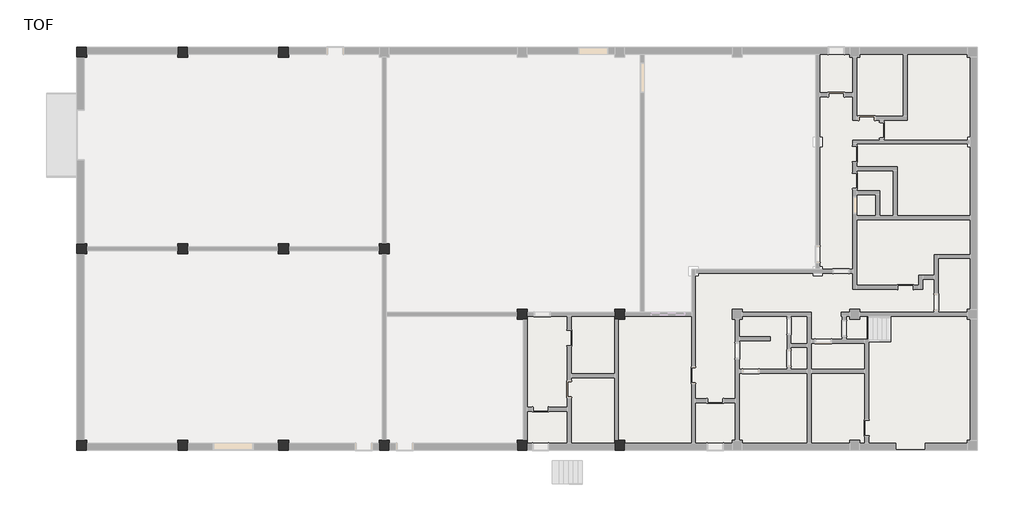
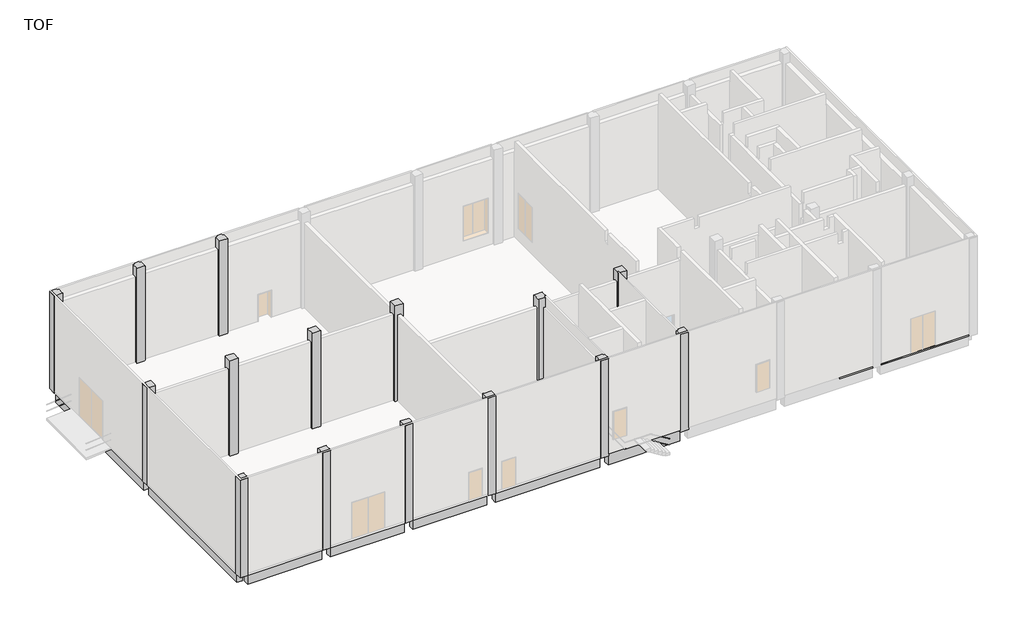
# One storey, part 4 of 5: 15 columns, 9 beams, 4 slabs.
"""IFC4 building model written with IfcOpenShell, lengths in millimetres."""

from ifc_helpers import new_model, si_unit, frame, origin, place, context, project, spatial, polyline, outline, extrude, faceted_brep, element, save

model = new_model("IFC4")

# Units and contexts
model_context = context("Model", 3, world=origin())
ifc_project = project(units=[si_unit("LENGTHUNIT", "METRE", prefix="MILLI")], contexts=[model_context])

# Site, building, storey
site = spatial("IfcSite", under=ifc_project)
building = spatial("IfcBuilding", under=site)
storey = spatial("IfcBuildingStorey", under=building, Name="TOF", Elevation=150.0)

# Beams
placement = place(None, origin())
element("IfcBeam", 1, ObjectType="RC Beam_Rectangular : H_SB_ACB_B400xH900", at=placement, inside=storey, context=model_context, shape_type="SweptSolid", body=[
    extrude(outline(polyline([(124.7, 12616.5208589), (-275.3, 12616.5208589), (-275.3, 23716.5208589), (124.7, 23716.5208589), (124.7, 12616.5208589)])), frame((0.0, 0.0, -750.0), z_axis=(0.0, 0.0, 1.0), x_axis=(1.0, 0.0, 0.0)), (0.0, 0.0, 1.0), 800.0),
])
element("IfcBeam", 2, ObjectType="RC Beam_Rectangular : H_SB_ACB_B400xH900", at=placement, inside=storey, context=model_context, shape_type="SweptSolid", body=[
    extrude(outline(polyline([(124.7, 916.5208589), (-275.3, 916.5208589), (-275.3, 12016.5208589), (124.7, 12016.5208589), (124.7, 916.5208589)])), frame((0.0, 0.0, -750.0), z_axis=(0.0, 0.0, 1.0), x_axis=(1.0, 0.0, 0.0)), (0.0, 0.0, 1.0), 750.0),
])
element("IfcBeam", 3, ObjectType="RC Beam_Rectangular : H_SB_ACB_B400xH900", at=placement, inside=storey, context=model_context, shape_type="SweptSolid", body=[
    extrude(outline(polyline([(5624.7, 24216.5208589), (5624.7, 23816.5208589), (224.7, 23816.5208589), (224.7, 24216.5208589), (5624.7, 24216.5208589)])), frame((0.0, 0.0, -750.0), z_axis=(0.0, 0.0, 1.0), x_axis=(1.0, 0.0, 0.0)), (0.0, 0.0, 1.0), 800.0),
])
element("IfcBeam", 4, ObjectType="RC Beam_Rectangular : H_SB_ACB_B400xH900", at=placement, inside=storey, context=model_context, shape_type="SweptSolid", body=[
    extrude(outline(polyline([(11624.7, 24216.5208589), (11624.7, 23816.5208589), (6224.7, 23816.5208589), (6224.7, 24216.5208589), (11624.7, 24216.5208589)])), frame((0.0, 0.0, -750.0), z_axis=(0.0, 0.0, 1.0), x_axis=(1.0, 0.0, 0.0)), (0.0, 0.0, 1.0), 800.0),
])
element("IfcBeam", 5, ObjectType="RC Beam_Rectangular : H_SB_ACB_B400xH900", at=placement, inside=storey, context=model_context, shape_type="SweptSolid", body=[
    extrude(outline(polyline([(5624.7, 816.5208589), (5624.7, 416.5208589), (224.7, 416.5208589), (224.7, 816.5208589), (5624.7, 816.5208589)])), frame((0.0, 0.0, -750.0), z_axis=(0.0, 0.0, 1.0), x_axis=(1.0, 0.0, 0.0)), (0.0, 0.0, 1.0), 750.0),
])
element("IfcBeam", 6, ObjectType="RC Beam_Rectangular : H_SB_ACB_B400xH900", at=placement, inside=storey, context=model_context, shape_type="SweptSolid", body=[
    extrude(outline(polyline([(11624.7, 816.5208589), (11624.7, 416.5208589), (6224.7, 416.5208589), (6224.7, 816.5208589), (11624.7, 816.5208589)])), frame((0.0, 0.0, -750.0), z_axis=(0.0, 0.0, 1.0), x_axis=(1.0, 0.0, 0.0)), (0.0, 0.0, 1.0), 750.0),
])
element("IfcBeam", 7, ObjectType="RC Beam_Rectangular : H_SB_ACB_B400xH900", at=placement, inside=storey, context=model_context, shape_type="SweptSolid", body=[
    extrude(outline(polyline([(17624.7, 816.5208589), (17624.7, 416.5208589), (12224.7, 416.5208589), (12224.7, 816.5208589), (17624.7, 816.5208589)])), frame((0.0, 0.0, -750.0), z_axis=(0.0, 0.0, 1.0), x_axis=(1.0, 0.0, 0.0)), (0.0, 0.0, 1.0), 750.0),
])
element("IfcBeam", 8, ObjectType="RC Beam_Rectangular : H_SB_ACB_B400xH900", at=placement, inside=storey, context=model_context, shape_type="SweptSolid", body=[
    extrude(outline(polyline([(25824.7, 816.5208589), (25824.7, 416.5208589), (18224.7, 416.5208589), (18224.7, 816.5208589), (25824.7, 816.5208589)])), frame((0.0, 0.0, -750.0), z_axis=(0.0, 0.0, 1.0), x_axis=(1.0, 0.0, 0.0)), (0.0, 0.0, 1.0), 750.0),
])
element("IfcBeam", 9, ObjectType="RC Beam_Rectangular : H_SB_ACB_B400xH900", at=placement, inside=storey, context=model_context, shape_type="Brep", body=[
    faceted_brep([(26424.7, 816.5208589, 150.0), (26424.7, 746.5208589, 150.0), (26424.7, 416.5208589, 150.0), (31624.7, 416.5208589, 150.0), (31624.7, 746.5208589, 150.0), (31624.7, 816.5208589, 150.0), (26424.7, 416.5208589, -750.0), (31624.7, 416.5208589, -750.0), (26424.7, 816.5208589, -750.0), (31624.7, 816.5208589, -750.0)], [[[0, 1, 2, 3, 4, 5]], [[2, 6, 7, 3]], [[6, 8, 9, 7]], [[8, 0, 5, 9]], [[2, 1, 0, 8, 6]], [[5, 4, 3, 7, 9]]]),
])

# Columns
element("IfcColumn", 10, ObjectType="RC_Column_Rectangular : H_SC_ACC_W600xL600", at=placement, inside=storey, context=model_context, shape_type="Brep", body=[
    faceted_brep([(224.7, 12616.5208589, 0.0), (224.7, 12316.5208589, 0.0), (224.7, 12016.5208589, 0.0), (-375.3, 12016.5208589, 0.0), (-375.3, 12616.5208589, 0.0), (224.7, 12616.5208589, 7500.0), (224.7, 12516.5208589, 7500.0), (224.7, 12116.5208589, 7500.0), (224.7, 12016.5208589, 7500.0), (224.7, 12016.5208589, 150.0), (224.7, 12616.5208589, 50.0), (224.7, 12616.5208589, 200.0), (124.7, 12016.5208589, 7500.0), (-275.3, 12016.5208589, 7500.0), (-375.3, 12016.5208589, 7500.0), (-375.3, 12016.5208589, 150.0), (-375.3, 12616.5208589, 7500.0), (-375.3, 12616.5208589, 150.0), (-375.3, 12616.5208589, 50.0), (-275.3, 12616.5208589, 7500.0), (124.7, 12616.5208589, 7500.0)], [[[0, 1, 2, 3, 4]], [[5, 6, 7, 8, 9, 2, 1, 0, 10, 11]], [[8, 12, 13, 14, 15, 3, 2, 9]], [[14, 16, 17, 18, 4, 3, 15]], [[16, 19, 20, 5, 11, 10, 0, 4, 18, 17]], [[5, 20, 19, 16, 14, 13, 12, 8, 7, 6]]]),
])
element("IfcColumn", 11, ObjectType="RC_Column_Rectangular : H_SC_ACC_W600xL600", at=placement, inside=storey, context=model_context, shape_type="Brep", body=[
    faceted_brep([(6224.7, 12616.5208589, 0.0), (6224.7, 12316.5208589, 0.0), (6224.7, 12016.5208589, 0.0), (5624.7, 12016.5208589, 0.0), (5624.7, 12316.5208589, 0.0), (5624.7, 12616.5208589, 0.0), (6224.7, 12616.5208589, 7500.0), (6224.7, 12516.5208589, 7500.0), (6224.7, 12116.5208589, 7500.0), (6224.7, 12016.5208589, 7500.0), (6224.7, 12016.5208589, 150.0), (6224.7, 12616.5208589, 50.0), (6224.7, 12616.5208589, 200.0), (6124.7, 12016.5208589, 7500.0), (5724.7, 12016.5208589, 7500.0), (5624.7, 12016.5208589, 7500.0), (5624.7, 12016.5208589, 150.0), (5624.7, 12116.5208589, 7500.0), (5624.7, 12516.5208589, 7500.0), (5624.7, 12616.5208589, 7500.0), (5624.7, 12616.5208589, 200.0), (5624.7, 12616.5208589, 50.0), (5724.7, 12616.5208589, 7500.0), (6124.7, 12616.5208589, 7500.0)], [[[0, 1, 2, 3, 4, 5]], [[6, 7, 8, 9, 10, 2, 1, 0, 11, 12]], [[9, 13, 14, 15, 16, 3, 2, 10]], [[15, 17, 18, 19, 20, 21, 5, 4, 3, 16]], [[19, 22, 23, 6, 12, 11, 0, 5, 21, 20]], [[6, 23, 22, 19, 18, 17, 15, 14, 13, 9, 8, 7]]]),
])
element("IfcColumn", 12, ObjectType="RC_Column_Rectangular : H_SC_ACC_W600xL600", at=placement, inside=storey, context=model_context, shape_type="Brep", body=[
    faceted_brep([(12224.7, 12616.5208589, 0.0), (12224.7, 12316.5208589, 0.0), (12224.7, 12016.5208589, 0.0), (11624.7, 12016.5208589, 0.0), (11624.7, 12316.5208589, 0.0), (11624.7, 12616.5208589, 0.0), (12224.7, 12616.5208589, 7500.0), (12224.7, 12516.5208589, 7500.0), (12224.7, 12116.5208589, 7500.0), (12224.7, 12016.5208589, 7500.0), (12224.7, 12016.5208589, 150.0), (12224.7, 12616.5208589, 50.0), (12224.7, 12616.5208589, 200.0), (12124.7, 12016.5208589, 7500.0), (11724.7, 12016.5208589, 7500.0), (11624.7, 12016.5208589, 7500.0), (11624.7, 12016.5208589, 150.0), (11624.7, 12116.5208589, 7500.0), (11624.7, 12516.5208589, 7500.0), (11624.7, 12616.5208589, 7500.0), (11624.7, 12616.5208589, 200.0), (11624.7, 12616.5208589, 50.0), (11724.7, 12616.5208589, 7500.0), (12124.7, 12616.5208589, 7500.0)], [[[0, 1, 2, 3, 4, 5]], [[6, 7, 8, 9, 10, 2, 1, 0, 11, 12]], [[9, 13, 14, 15, 16, 3, 2, 10]], [[15, 17, 18, 19, 20, 21, 5, 4, 3, 16]], [[19, 22, 23, 6, 12, 11, 0, 5, 21, 20]], [[6, 23, 22, 19, 18, 17, 15, 14, 13, 9, 8, 7]]]),
])
element("IfcColumn", 13, ObjectType="RC_Column_Rectangular : H_SC_ACC_W600xL600", at=placement, inside=storey, context=model_context, shape_type="Brep", body=[
    faceted_brep([(18224.7, 12616.5208589, 0.0), (18224.7, 12016.5208589, 0.0), (17924.7, 12016.5208589, 0.0), (17624.7, 12016.5208589, 0.0), (17624.7, 12316.5208589, 0.0), (17624.7, 12616.5208589, 0.0), (18224.7, 12616.5208589, 7500.0), (18224.7, 12516.5208589, 7500.0), (18224.7, 12116.5208589, 7500.0), (18224.7, 12016.5208589, 7500.0), (18224.7, 12016.5208589, 200.0), (18224.7, 12016.5208589, 50.0), (18224.7, 12616.5208589, 50.0), (18224.7, 12616.5208589, 200.0), (18124.7, 12016.5208589, 7500.0), (17724.7, 12016.5208589, 7500.0), (17624.7, 12016.5208589, 7500.0), (17624.7, 12016.5208589, 150.0), (17624.7, 12116.5208589, 7500.0), (17624.7, 12516.5208589, 7500.0), (17624.7, 12616.5208589, 7500.0), (17624.7, 12616.5208589, 200.0), (17624.7, 12616.5208589, 50.0), (17724.7, 12616.5208589, 7500.0), (18124.7, 12616.5208589, 7500.0)], [[[0, 1, 2, 3, 4, 5]], [[6, 7, 8, 9, 10, 11, 1, 0, 12, 13]], [[9, 14, 15, 16, 17, 3, 2, 1, 11, 10]], [[16, 18, 19, 20, 21, 22, 5, 4, 3, 17]], [[20, 23, 24, 6, 13, 12, 0, 5, 22, 21]], [[6, 24, 23, 20, 19, 18, 16, 15, 14, 9, 8, 7]]]),
])
element("IfcColumn", 14, ObjectType="RC_Column_Rectangular : H_SC_ACC_W600xL600", at=placement, inside=storey, context=model_context, shape_type="Brep", body=[
    faceted_brep([(224.7, 24316.5208589, 0.0), (224.7, 23716.5208589, 0.0), (-375.3, 23716.5208589, 0.0), (-375.3, 24316.5208589, 0.0), (224.7, 24316.5208589, 7500.0), (224.7, 24216.5208589, 7500.0), (224.7, 23816.5208589, 7500.0), (224.7, 23716.5208589, 7500.0), (224.7, 23716.5208589, 200.0), (224.7, 23716.5208589, 50.0), (224.7, 24316.5208589, 50.0), (224.7, 24316.5208589, 150.0), (124.7, 23716.5208589, 7500.0), (-275.3, 23716.5208589, 7500.0), (-375.3, 23716.5208589, 7500.0), (-375.3, 23716.5208589, 150.0), (-375.3, 23716.5208589, 50.0), (-375.3, 23886.5208589, 7500.0), (-375.3, 24316.5208589, 7500.0), (-275.3, 24316.5208589, 7500.0), (124.7, 24316.5208589, 7500.0)], [[[0, 1, 2, 3]], [[4, 5, 6, 7, 8, 9, 1, 0, 10, 11]], [[7, 12, 13, 14, 15, 16, 2, 1, 9, 8]], [[14, 17, 18, 3, 2, 16, 15]], [[18, 19, 20, 4, 11, 10, 0, 3]], [[4, 20, 19, 18, 17, 14, 13, 12, 7, 6, 5]]]),
])
element("IfcColumn", 15, ObjectType="RC_Column_Rectangular : H_SC_ACC_W600xL600", at=placement, inside=storey, context=model_context, shape_type="Brep", body=[
    faceted_brep([(6224.7, 24316.5208589, 0.0), (6224.7, 23716.5208589, 0.0), (5624.7, 23716.5208589, 0.0), (5624.7, 24316.5208589, 0.0), (6224.7, 24316.5208589, 7500.0), (6224.7, 24216.5208589, 7500.0), (6224.7, 23816.5208589, 7500.0), (6224.7, 23716.5208589, 7500.0), (6224.7, 23716.5208589, 200.0), (6224.7, 23716.5208589, 50.0), (6224.7, 24316.5208589, 50.0), (6224.7, 24316.5208589, 150.0), (6124.7, 23716.5208589, 7500.0), (5724.7, 23716.5208589, 7500.0), (5624.7, 23716.5208589, 7500.0), (5624.7, 23716.5208589, 200.0), (5624.7, 23716.5208589, 50.0), (5624.7, 23816.5208589, 7500.0), (5624.7, 24216.5208589, 7500.0), (5624.7, 24316.5208589, 7500.0), (5624.7, 24316.5208589, 150.0), (5624.7, 24316.5208589, 50.0), (5724.7, 24316.5208589, 7500.0), (6124.7, 24316.5208589, 7500.0)], [[[0, 1, 2, 3]], [[4, 5, 6, 7, 8, 9, 1, 0, 10, 11]], [[7, 12, 13, 14, 15, 16, 2, 1, 9, 8]], [[14, 17, 18, 19, 20, 21, 3, 2, 16, 15]], [[19, 22, 23, 4, 11, 10, 0, 3, 21, 20]], [[4, 23, 22, 19, 18, 17, 14, 13, 12, 7, 6, 5]]]),
])
element("IfcColumn", 16, ObjectType="RC_Column_Rectangular : H_SC_ACC_W600xL600", at=placement, inside=storey, context=model_context, shape_type="Brep", body=[
    faceted_brep([(12224.7, 24316.5208589, 0.0), (12224.7, 23716.5208589, 0.0), (11624.7, 23716.5208589, 0.0), (11624.7, 24316.5208589, 0.0), (12224.7, 24316.5208589, 7500.0), (12224.7, 24216.5208589, 7500.0), (12224.7, 23816.5208589, 7500.0), (12224.7, 23716.5208589, 7500.0), (12224.7, 23716.5208589, 200.0), (12224.7, 23716.5208589, 50.0), (12224.7, 24316.5208589, 50.0), (12224.7, 24316.5208589, 150.0), (12124.7, 23716.5208589, 7500.0), (11724.7, 23716.5208589, 7500.0), (11624.7, 23716.5208589, 7500.0), (11624.7, 23716.5208589, 200.0), (11624.7, 23716.5208589, 50.0), (11624.7, 23816.5208589, 7500.0), (11624.7, 24216.5208589, 7500.0), (11624.7, 24316.5208589, 7500.0), (11624.7, 24316.5208589, 150.0), (11624.7, 24316.5208589, 50.0), (11724.7, 24316.5208589, 7500.0), (12124.7, 24316.5208589, 7500.0)], [[[0, 1, 2, 3]], [[4, 5, 6, 7, 8, 9, 1, 0, 10, 11]], [[7, 12, 13, 14, 15, 16, 2, 1, 9, 8]], [[14, 17, 18, 19, 20, 21, 3, 2, 16, 15]], [[19, 22, 23, 4, 11, 10, 0, 3, 21, 20]], [[4, 23, 22, 19, 18, 17, 14, 13, 12, 7, 6, 5]]]),
])
element("IfcColumn", 17, ObjectType="RC_Column_Rectangular : H_SC_ACC_W600xL600", at=placement, inside=storey, context=model_context, shape_type="Brep", body=[
    faceted_brep([(26424.7, 8716.5208589, 0.0), (26424.7, 8116.5208589, 0.0), (26307.7, 8116.5208589, 0.0), (25824.7, 8116.5208589, 0.0), (25824.7, 8416.5208589, 0.0), (25824.7, 8716.5208589, 0.0), (26424.7, 8716.5208589, 7500.0), (26424.7, 8616.5208589, 7500.0), (26424.7, 8216.5208589, 7500.0), (26424.7, 8116.5208589, 7500.0), (26424.7, 8116.5208589, 150.0), (26424.7, 8716.5208589, 50.0), (26424.7, 8716.5208589, 200.0), (26324.7, 8116.5208589, 7500.0), (25924.7, 8116.5208589, 7500.0), (25824.7, 8116.5208589, 7500.0), (25824.7, 8116.5208589, 150.0), (25824.7, 8216.5208589, 7500.0), (25824.7, 8616.5208589, 7500.0), (25824.7, 8716.5208589, 7500.0), (25824.7, 8716.5208589, 200.0), (25824.7, 8716.5208589, 50.0), (25924.7, 8716.5208589, 7500.0), (26324.7, 8716.5208589, 7500.0)], [[[0, 1, 2, 3, 4, 5]], [[6, 7, 8, 9, 10, 1, 0, 11, 12]], [[9, 13, 14, 15, 16, 3, 2, 1, 10]], [[15, 17, 18, 19, 20, 21, 5, 4, 3, 16]], [[19, 22, 23, 6, 12, 11, 0, 5, 21, 20]], [[6, 23, 22, 19, 18, 17, 15, 14, 13, 9, 8, 7]]]),
])
element("IfcColumn", 18, ObjectType="RC_Column_Rectangular : H_SC_ACC_W600xL600", at=placement, inside=storey, context=model_context, shape_type="Brep", body=[
    faceted_brep([(32224.7, 8716.5208589, 0.0), (32224.7, 8116.5208589, 0.0), (31624.7, 8116.5208589, 0.0), (31624.7, 8716.5208589, 0.0), (32224.7, 8716.5208589, 7500.0), (32224.7, 8616.5208589, 7500.0), (32224.7, 8216.5208589, 7500.0), (32224.7, 8116.5208589, 7500.0), (32224.7, 8116.5208589, 1150.0), (32224.7, 8116.5208589, 1000.0), (32224.7, 8716.5208589, 50.0), (32224.7, 8716.5208589, 200.0), (32124.7, 8116.5208589, 7500.0), (31724.7, 8116.5208589, 7500.0), (31624.7, 8116.5208589, 7500.0), (31624.7, 8116.5208589, 1150.0), (31624.7, 8116.5208589, 1000.0), (31624.7, 8216.5208589, 7500.0), (31624.7, 8616.5208589, 7500.0), (31624.7, 8716.5208589, 7500.0), (31624.7, 8716.5208589, 200.0), (31624.7, 8716.5208589, 50.0), (31724.7, 8716.5208589, 7500.0), (32124.7, 8716.5208589, 7500.0)], [[[0, 1, 2, 3]], [[4, 5, 6, 7, 8, 9, 1, 0, 10, 11]], [[7, 12, 13, 14, 15, 16, 2, 1, 9, 8]], [[14, 17, 18, 19, 20, 21, 3, 2, 16, 15]], [[19, 22, 23, 4, 11, 10, 0, 3, 21, 20]], [[4, 23, 22, 19, 18, 17, 14, 13, 12, 7, 6, 5]]]),
])
element("IfcColumn", 19, ObjectType="RC_Column_Rectangular : H_SC_ACC_W600xL600", at=placement, inside=storey, context=model_context, shape_type="Brep", body=[
    faceted_brep([(224.7, 916.5208589, 0.0), (224.7, 316.5208589, 0.0), (-375.3, 316.5208589, 0.0), (-375.3, 916.5208589, 0.0), (224.7, 916.5208589, 7500.0), (224.7, 816.5208589, 7500.0), (224.7, 416.5208589, 7500.0), (224.7, 316.5208589, 7500.0), (224.7, 316.5208589, 150.0), (224.7, 916.5208589, 150.0), (54.7, 316.5208589, 7500.0), (-375.3, 316.5208589, 7500.0), (-375.3, 916.5208589, 7500.0), (-375.3, 916.5208589, 150.0), (-275.3, 916.5208589, 7500.0), (124.7, 916.5208589, 7500.0)], [[[0, 1, 2, 3]], [[4, 5, 6, 7, 8, 1, 0, 9]], [[7, 10, 11, 2, 1, 8]], [[11, 12, 13, 3, 2]], [[12, 14, 15, 4, 9, 0, 3, 13]], [[4, 15, 14, 12, 11, 10, 7, 6, 5]]]),
])
element("IfcColumn", 20, ObjectType="RC_Column_Rectangular : H_SC_ACC_W600xL600", at=placement, inside=storey, context=model_context, shape_type="Brep", body=[
    faceted_brep([(6224.7, 916.5208589, 0.0), (6224.7, 316.5208589, 0.0), (5624.7, 316.5208589, 0.0), (5624.7, 916.5208589, 0.0), (6224.7, 916.5208589, 7500.0), (6224.7, 816.5208589, 7500.0), (6224.7, 416.5208589, 7500.0), (6224.7, 316.5208589, 7500.0), (6224.7, 316.5208589, 150.0), (6224.7, 916.5208589, 150.0), (5624.7, 316.5208589, 7500.0), (5624.7, 316.5208589, 150.0), (5624.7, 416.5208589, 7500.0), (5624.7, 816.5208589, 7500.0), (5624.7, 916.5208589, 7500.0), (5624.7, 916.5208589, 150.0), (5724.7, 916.5208589, 7500.0), (6124.7, 916.5208589, 7500.0)], [[[0, 1, 2, 3]], [[4, 5, 6, 7, 8, 1, 0, 9]], [[7, 10, 11, 2, 1, 8]], [[10, 12, 13, 14, 15, 3, 2, 11]], [[14, 16, 17, 4, 9, 0, 3, 15]], [[4, 17, 16, 14, 13, 12, 10, 7, 6, 5]]]),
])
element("IfcColumn", 21, ObjectType="RC_Column_Rectangular : H_SC_ACC_W600xL600", at=placement, inside=storey, context=model_context, shape_type="Brep", body=[
    faceted_brep([(12224.7, 916.5208589, 0.0), (12224.7, 316.5208589, 0.0), (11624.7, 316.5208589, 0.0), (11624.7, 916.5208589, 0.0), (12224.7, 916.5208589, 7500.0), (12224.7, 816.5208589, 7500.0), (12224.7, 416.5208589, 7500.0), (12224.7, 316.5208589, 7500.0), (12224.7, 316.5208589, 150.0), (12224.7, 916.5208589, 150.0), (11624.7, 316.5208589, 7500.0), (11624.7, 316.5208589, 150.0), (11624.7, 416.5208589, 7500.0), (11624.7, 816.5208589, 7500.0), (11624.7, 916.5208589, 7500.0), (11624.7, 916.5208589, 150.0), (11724.7, 916.5208589, 7500.0), (12124.7, 916.5208589, 7500.0)], [[[0, 1, 2, 3]], [[4, 5, 6, 7, 8, 1, 0, 9]], [[7, 10, 11, 2, 1, 8]], [[10, 12, 13, 14, 15, 3, 2, 11]], [[14, 16, 17, 4, 9, 0, 3, 15]], [[4, 17, 16, 14, 13, 12, 10, 7, 6, 5]]]),
])
element("IfcColumn", 22, ObjectType="RC_Column_Rectangular : H_SC_ACC_W600xL600", at=placement, inside=storey, context=model_context, shape_type="Brep", body=[
    faceted_brep([(18224.7, 916.5208589, 0.0), (18224.7, 316.5208589, 0.0), (17624.7, 316.5208589, 0.0), (17624.7, 916.5208589, 0.0), (18224.7, 916.5208589, 7500.0), (18224.7, 816.5208589, 7500.0), (18224.7, 416.5208589, 7500.0), (18224.7, 316.5208589, 7500.0), (18224.7, 316.5208589, 150.0), (18224.7, 916.5208589, 150.0), (17624.7, 316.5208589, 7500.0), (17624.7, 316.5208589, 150.0), (17624.7, 416.5208589, 7500.0), (17624.7, 816.5208589, 7500.0), (17624.7, 916.5208589, 7500.0), (17624.7, 916.5208589, 150.0), (17724.7, 916.5208589, 7500.0), (18124.7, 916.5208589, 7500.0)], [[[0, 1, 2, 3]], [[4, 5, 6, 7, 8, 1, 0, 9]], [[7, 10, 11, 2, 1, 8]], [[10, 12, 13, 14, 15, 3, 2, 11]], [[14, 16, 17, 4, 9, 0, 3, 15]], [[4, 17, 16, 14, 13, 12, 10, 7, 6, 5]]]),
])
element("IfcColumn", 23, ObjectType="RC_Column_Rectangular : H_SC_ACC_W600xL600", at=placement, inside=storey, context=model_context, shape_type="Brep", body=[
    faceted_brep([(26424.7, 916.5208589, 0.0), (26424.7, 316.5208589, 0.0), (25824.7, 316.5208589, 0.0), (25824.7, 916.5208589, 0.0), (26307.7, 916.5208589, 0.0), (26424.7, 916.5208589, 7500.0), (26424.7, 816.5208589, 7500.0), (26424.7, 416.5208589, 7500.0), (26424.7, 316.5208589, 7500.0), (26424.7, 316.5208589, 150.0), (26424.7, 916.5208589, 150.0), (25824.7, 316.5208589, 7500.0), (25824.7, 316.5208589, 150.0), (25824.7, 416.5208589, 7500.0), (25824.7, 816.5208589, 7500.0), (25824.7, 916.5208589, 7500.0), (25824.7, 916.5208589, 150.0), (25924.7, 916.5208589, 7500.0), (26324.7, 916.5208589, 7500.0)], [[[0, 1, 2, 3, 4]], [[5, 6, 7, 8, 9, 1, 0, 10]], [[8, 11, 12, 2, 1, 9]], [[11, 13, 14, 15, 16, 3, 2, 12]], [[15, 17, 18, 5, 10, 0, 4, 3, 16]], [[5, 18, 17, 15, 14, 13, 11, 8, 7, 6]]]),
])
element("IfcColumn", 24, ObjectType="RC_Column_Rectangular : H_SC_ACC_W600xL600", at=placement, inside=storey, context=model_context, shape_type="Brep", body=[
    faceted_brep([(32224.7, 916.5208589, 0.0), (32224.7, 316.5208589, 0.0), (31624.7, 316.5208589, 0.0), (31624.7, 916.5208589, 0.0), (32224.7, 916.5208589, 7500.0), (32224.7, 816.5208589, 7500.0), (32224.7, 416.5208589, 7500.0), (32224.7, 316.5208589, 7500.0), (32224.7, 316.5208589, 150.0), (32224.7, 916.5208589, 1000.0), (32224.7, 916.5208589, 1150.0), (31624.7, 316.5208589, 7500.0), (31624.7, 316.5208589, 150.0), (31624.7, 416.5208589, 7500.0), (31624.7, 816.5208589, 7500.0), (31624.7, 916.5208589, 7500.0), (31624.7, 916.5208589, 1150.0), (31624.7, 916.5208589, 1000.0), (31724.7, 916.5208589, 7500.0), (32124.7, 916.5208589, 7500.0)], [[[0, 1, 2, 3]], [[4, 5, 6, 7, 8, 1, 0, 9, 10]], [[7, 11, 12, 2, 1, 8]], [[11, 13, 14, 15, 16, 17, 3, 2, 12]], [[15, 18, 19, 4, 10, 9, 0, 3, 17, 16]], [[4, 19, 18, 15, 14, 13, 11, 7, 6, 5]]]),
])

# Slabs
element("IfcSlab", 25, ObjectType="H_FL_AMF_RC Slab_T150", at=placement, inside=storey, context=model_context, shape_type="Brep", body=[
    faceted_brep([(45624.7, 23716.5208589, 1000.0), (46224.7, 23716.5208589, 1000.0), (46224.7, 23886.5208589, 1000.0), (52624.7, 23886.5208589, 1000.0), (52624.7, 23716.5208589, 1000.0), (52794.7, 23716.5208589, 1000.0), (52794.7, 18966.5208589, 1000.0), (52624.7, 18966.5208589, 1000.0), (52624.7, 18366.5208589, 1000.0), (52794.7, 18366.5208589, 1000.0), (52794.7, 11850.5208589, 1000.0), (50894.7, 11850.5208589, 1000.0), (50894.7, 11967.5208589, 1000.0), (50660.7, 11967.5208589, 1000.0), (50660.7, 8533.5208589, 1000.0), (46224.7, 8533.5208589, 1000.0), (46224.7, 8716.5208589, 1000.0), (45624.7, 8716.5208589, 1000.0), (45624.7, 8533.5208589, 1000.0), (45124.7, 8533.5208589, 1000.0), (45124.7, 8299.5208589, 1000.0), (45175.8778017, 8299.5208589, 1000.0), (45175.8778017, 6933.5208589, 1000.0), (43341.7, 6933.5208589, 1000.0), (43341.7, 8533.5208589, 1000.0), (39224.7, 8533.5208589, 1000.0), (39224.7, 8716.5208589, 1000.0), (38624.7, 8716.5208589, 1000.0), (38624.7, 8116.5208589, 1000.0), (38807.7, 8116.5208589, 1000.0), (38807.7, 916.5208589, 1000.0), (38624.7, 916.5208589, 1000.0), (38624.7, 746.5208589, 1000.0), (32224.7, 746.5208589, 1000.0), (32224.7, 916.5208589, 1000.0), (31624.7, 916.5208589, 1000.0), (31624.7, 746.5208589, 1000.0), (26424.7, 746.5208589, 1000.0), (26424.7, 8299.5208589, 1000.0), (31624.7, 8299.5208589, 1000.0), (31624.7, 8116.5208589, 1000.0), (32224.7, 8116.5208589, 1000.0), (32224.7, 8299.5208589, 1000.0), (36207.7, 8299.5208589, 1000.0), (36207.7, 8416.5208589, 1000.0), (36324.7, 8416.5208589, 1000.0), (36324.7, 10666.5208589, 1000.0), (36624.7, 10666.5208589, 1000.0), (36624.7, 10849.5208589, 1000.0), (43424.7, 10849.5208589, 1000.0), (43424.7, 10666.5208589, 1000.0), (44024.7, 10666.5208589, 1000.0), (44024.7, 10849.5208589, 1000.0), (45807.7, 10849.5208589, 1000.0), (45807.7, 11083.5208589, 1000.0), (44024.7, 11083.5208589, 1000.0), (44024.7, 11266.5208589, 1000.0), (43841.7, 11266.5208589, 1000.0), (43841.7, 18366.5208589, 1000.0), (44024.7, 18366.5208589, 1000.0), (44024.7, 18966.5208589, 1000.0), (43841.7, 18966.5208589, 1000.0), (43841.7, 23886.5208589, 1000.0), (45624.7, 23886.5208589, 1000.0), (46224.7, 23716.5208589, 1150.0), (46041.7, 23716.5208589, 1150.0), (45807.7, 23716.5208589, 1150.0), (45624.7, 23716.5208589, 1150.0), (45624.7, 23886.5208589, 1150.0), (45324.7, 23886.5208589, 1150.0), (44324.7, 23886.5208589, 1150.0), (43841.7, 23886.5208589, 1150.0), (43841.7, 21586.5208589, 1150.0), (43841.7, 21352.5208589, 1150.0), (43841.7, 18966.5208589, 1150.0), (44024.7, 18966.5208589, 1150.0), (44024.7, 18366.5208589, 1150.0), (43841.7, 18366.5208589, 1150.0), (43841.7, 12483.5208589, 1150.0), (43841.7, 11483.5208589, 1150.0), (43841.7, 11266.5208589, 1150.0), (44024.7, 11266.5208589, 1150.0), (44024.7, 11083.5208589, 1150.0), (44607.7, 11083.5208589, 1150.0), (45607.7, 11083.5208589, 1150.0), (45807.7, 11083.5208589, 1150.0), (45807.7, 10849.5208589, 1150.0), (45607.7, 10849.5208589, 1150.0), (44607.7, 10849.5208589, 1150.0), (44024.7, 10849.5208589, 1150.0), (44024.7, 10666.5208589, 1150.0), (43424.7, 10666.5208589, 1150.0), (43424.7, 10849.5208589, 1150.0), (36624.7, 10849.5208589, 1150.0), (36624.7, 10666.5208589, 1150.0), (36324.7, 10666.5208589, 1150.0), (36324.7, 8416.5208589, 1150.0), (36207.7, 8416.5208589, 1150.0), (36207.7, 8299.5208589, 1150.0), (32224.7, 8299.5208589, 1150.0), (32224.7, 8116.5208589, 1150.0), (31858.7, 8116.5208589, 1150.0), (31624.7, 8116.5208589, 1150.0), (31624.7, 8299.5208589, 1150.0), (29058.7, 8299.5208589, 1150.0), (28824.7, 8299.5208589, 1150.0), (27824.7, 8299.5208589, 1150.0), (26824.7, 8299.5208589, 1150.0), (26424.7, 8299.5208589, 1150.0), (26424.7, 2880.5208589, 1150.0), (26424.7, 2646.5208589, 1150.0), (26424.7, 746.5208589, 1150.0), (26724.7, 746.5208589, 1150.0), (27724.7, 746.5208589, 1150.0), (28824.7, 746.5208589, 1150.0), (29058.7, 746.5208589, 1150.0), (31624.7, 746.5208589, 1150.0), (31624.7, 916.5208589, 1150.0), (31858.7, 916.5208589, 1150.0), (32224.7, 916.5208589, 1150.0), (32224.7, 746.5208589, 1150.0), (36207.7, 746.5208589, 1150.0), (36441.7, 746.5208589, 1150.0), (37124.7, 746.5208589, 1150.0), (38124.7, 746.5208589, 1150.0), (38624.7, 746.5208589, 1150.0), (38624.7, 916.5208589, 1150.0), (38807.7, 916.5208589, 1150.0), (38807.7, 3146.5208589, 1150.0), (38807.7, 3380.5208589, 1150.0), (38807.7, 5746.5208589, 1150.0), (38807.7, 6746.5208589, 1150.0), (38807.7, 8116.5208589, 1150.0), (38624.7, 8116.5208589, 1150.0), (38624.7, 8716.5208589, 1150.0), (39224.7, 8716.5208589, 1150.0), (39224.7, 8533.5208589, 1150.0), (43341.7, 8533.5208589, 1150.0), (43341.7, 6933.5208589, 1150.0), (43541.7, 6933.5208589, 1150.0), (44541.7, 6933.5208589, 1150.0), (45175.8778017, 6933.5208589, 1150.0), (45175.8778017, 7071.4042881, 1150.0), (45175.8778017, 8071.4042881, 1150.0), (45175.8778017, 8299.5208589, 1150.0), (45124.7, 8299.5208589, 1150.0), (45124.7, 8533.5208589, 1150.0), (45624.7, 8533.5208589, 1150.0), (45624.7, 8716.5208589, 1150.0), (46224.7, 8716.5208589, 1150.0), (46224.7, 8533.5208589, 1150.0), (50660.7, 8533.5208589, 1150.0), (50660.7, 8633.5208589, 1150.0), (50660.7, 9633.5208589, 1150.0), (50660.7, 10499.5208589, 1150.0), (50660.7, 10733.5208589, 1150.0), (50660.7, 11967.5208589, 1150.0), (50894.7, 11967.5208589, 1150.0), (50894.7, 11850.5208589, 1150.0), (52794.7, 11850.5208589, 1150.0), (52794.7, 11967.5208589, 1150.0), (52794.7, 14049.5208589, 1150.0), (52794.7, 14283.5208589, 1150.0), (52794.7, 18366.5208589, 1150.0), (52624.7, 18366.5208589, 1150.0), (52624.7, 18966.5208589, 1150.0), (52794.7, 18966.5208589, 1150.0), (52794.7, 23716.5208589, 1150.0), (52624.7, 23716.5208589, 1150.0), (52624.7, 23886.5208589, 1150.0), (49041.7, 23886.5208589, 1150.0), (48807.7, 23886.5208589, 1150.0), (46224.7, 23886.5208589, 1150.0)], [[[0, 1, 2, 3, 4, 5, 6, 7, 8, 9, 10, 11, 12, 13, 14, 15, 16, 17, 18, 19, 20, 21, 22, 23, 24, 25, 26, 27, 28, 29, 30, 31, 32, 33, 34, 35, 36, 37, 38, 39, 40, 41, 42, 43, 44, 45, 46, 47, 48, 49, 50, 51, 52, 53, 54, 55, 56, 57, 58, 59, 60, 61, 62, 63]], [[64, 65, 66, 67, 68, 69, 70, 71, 72, 73, 74, 75, 76, 77, 78, 79, 80, 81, 82, 83, 84, 85, 86, 87, 88, 89, 90, 91, 92, 93, 94, 95, 96, 97, 98, 99, 100, 101, 102, 103, 104, 105, 106, 107, 108, 109, 110, 111, 112, 113, 114, 115, 116, 117, 118, 119, 120, 121, 122, 123, 124, 125, 126, 127, 128, 129, 130, 131, 132, 133, 134, 135, 136, 137, 138, 139, 140, 141, 142, 143, 144, 145, 146, 147, 148, 149, 150, 151, 152, 153, 154, 155, 156, 157, 158, 159, 160, 161, 162, 163, 164, 165, 166, 167, 168, 169, 170, 171, 172]], [[10, 159, 158, 11]], [[96, 45, 44, 97]], [[45, 96, 95, 46]], [[1, 64, 172, 2]], [[64, 1, 0, 67, 66, 65]], [[67, 0, 63, 68]], [[4, 168, 167, 5]], [[168, 4, 3, 169]], [[37, 111, 110, 109, 108, 38]], [[41, 100, 99, 42]], [[100, 41, 40, 102, 101]], [[102, 40, 39, 103]], [[135, 26, 25, 136]], [[28, 133, 132, 29]], [[133, 28, 27, 134]], [[134, 27, 26, 135]], [[149, 16, 15, 150]], [[17, 148, 147, 18]], [[148, 17, 16, 149]], [[119, 34, 33, 120]], [[35, 117, 116, 36]], [[117, 35, 34, 119, 118]], [[31, 126, 125, 32]], [[126, 31, 30, 127]], [[47, 94, 93, 48]], [[94, 47, 46, 95]], [[51, 90, 89, 52]], [[81, 56, 55, 82]], [[90, 51, 50, 91]], [[91, 50, 49, 92]], [[56, 81, 80, 57]], [[59, 76, 75, 60]], [[76, 59, 58, 77]], [[60, 75, 74, 61]], [[8, 164, 163, 9]], [[164, 8, 7, 165]], [[165, 7, 6, 166]], [[3, 2, 172, 171, 170, 169]], [[69, 68, 63, 62, 71, 70]], [[33, 32, 125, 124, 123, 122, 121, 120]], [[37, 36, 116, 115, 114, 113, 112, 111]], [[10, 9, 163, 162, 161, 160, 159]], [[6, 5, 167, 166]], [[39, 38, 108, 107, 106, 105, 104, 103]], [[98, 43, 42, 99]], [[43, 98, 97, 44]], [[49, 48, 93, 92]], [[86, 53, 52, 89, 88, 87]], [[54, 85, 84, 83, 82, 55]], [[53, 86, 85, 54]], [[58, 57, 80, 79, 78, 77]], [[62, 61, 74, 73, 72, 71]], [[13, 156, 155, 154, 153, 152, 151, 14]], [[157, 12, 11, 158]], [[156, 13, 12, 157]], [[138, 23, 22, 141, 140, 139]], [[15, 14, 151, 150]], [[146, 19, 18, 147]], [[20, 145, 144, 21]], [[19, 146, 145, 20]], [[30, 29, 132, 131, 130, 129, 128, 127]], [[24, 137, 136, 25]], [[137, 24, 23, 138]], [[22, 21, 144, 143, 142, 141]]]),
    faceted_brep([(45624.7, 8116.5208589, 1000.0), (46224.7, 8116.5208589, 1000.0), (46224.7, 8299.5208589, 1000.0), (46624.7, 8299.5208589, 1000.0), (46624.7, 6933.5208589, 1000.0), (45409.8778017, 6933.5208589, 1000.0), (45409.8778017, 8299.5208589, 1000.0), (45624.7, 8299.5208589, 1000.0), (46224.7, 8116.5208589, 1150.0), (45624.7, 8116.5208589, 1150.0), (45624.7, 8299.5208589, 1150.0), (45409.8778017, 8299.5208589, 1150.0), (45409.8778017, 8071.4042881, 1150.0), (45409.8778017, 7071.4042881, 1150.0), (45409.8778017, 6933.5208589, 1150.0), (46624.7, 6933.5208589, 1150.0), (46624.7, 8299.5208589, 1150.0), (46224.7, 8299.5208589, 1150.0)], [[[0, 1, 2, 3, 4, 5, 6, 7]], [[8, 9, 10, 11, 12, 13, 14, 15, 16, 17]], [[15, 4, 3, 16]], [[1, 8, 17, 2]], [[8, 1, 0, 9]], [[9, 0, 7, 10]], [[4, 15, 14, 5]], [[3, 2, 17, 16]], [[10, 7, 6, 11]], [[6, 5, 14, 13, 12, 11]]]),
    faceted_brep([(43341.7, 6699.5208589, 1000.0), (46507.7, 6699.5208589, 1000.0), (46507.7, 5130.5208589, 1000.0), (43341.7, 5130.5208589, 1000.0), (46507.7, 6699.5208589, 1150.0), (44541.7, 6699.5208589, 1150.0), (43541.7, 6699.5208589, 1150.0), (43341.7, 6699.5208589, 1150.0), (43341.7, 5130.5208589, 1150.0), (46507.7, 5130.5208589, 1150.0)], [[[0, 1, 2, 3]], [[4, 5, 6, 7, 8, 9]], [[1, 4, 9, 2]], [[1, 0, 7, 6, 5, 4]], [[7, 0, 3, 8]], [[3, 2, 9, 8]]]),
])
element("IfcSlab", 26, ObjectType="H_FL_AMF_RC Slab_T150", at=placement, inside=storey, context=model_context, shape_type="Brep", body=[
    faceted_brep([(52794.7, 8716.5208589, 1000.0), (52624.7, 8716.5208589, 1000.0), (52624.7, 8533.5208589, 1000.0), (50894.7, 8533.5208589, 1000.0), (50894.7, 11850.5208589, 1000.0), (52794.7, 11850.5208589, 1000.0), (52624.7, 8716.5208589, 1150.0), (52794.7, 8716.5208589, 1150.0), (52794.7, 11733.5208589, 1150.0), (52794.7, 11850.5208589, 1150.0), (50894.7, 11850.5208589, 1150.0), (50894.7, 11733.5208589, 1150.0), (50894.7, 9633.5208589, 1150.0), (50894.7, 8633.5208589, 1150.0), (50894.7, 8533.5208589, 1150.0), (52624.7, 8533.5208589, 1150.0)], [[[0, 1, 2, 3, 4, 5]], [[6, 7, 8, 9, 10, 11, 12, 13, 14, 15]], [[9, 5, 4, 10]], [[1, 6, 15, 2]], [[6, 1, 0, 7]], [[0, 5, 9, 8, 7]], [[4, 3, 14, 13, 12, 11, 10]], [[3, 2, 15, 14]]]),
])
element("IfcSlab", 27, ObjectType="H_FL_AMF_RC Slab_T150", at=placement, inside=storey, context=model_context, shape_type="Brep", body=[
    faceted_brep([(43224.7, 316.5208589, 50.0), (43224.7, 416.5208589, 50.0), (43224.7, 816.5208589, 50.0), (43224.7, 5018.5208589, 50.0), (46624.7, 5018.5208589, 50.0), (46624.7, 8416.5208589, 50.0), (52624.7, 8416.5208589, 50.0), (52624.7, 8116.5208589, 50.0), (52724.7, 8116.5208589, 50.0), (53124.7, 8116.5208589, 50.0), (53224.7, 8116.5208589, 50.0), (53224.7, 916.5208589, 50.0), (53124.7, 916.5208589, 50.0), (52724.7, 916.5208589, 50.0), (52624.7, 916.5208589, 50.0), (52624.7, 816.5208589, 50.0), (52624.7, 416.5208589, 50.0), (52624.7, 316.5208589, 50.0), (46224.7, 316.5208589, 50.0), (46224.7, 416.5208589, 50.0), (46224.7, 816.5208589, 50.0), (46224.7, 916.5208589, 50.0), (45624.7, 916.5208589, 50.0), (45624.7, 816.5208589, 50.0), (45624.7, 416.5208589, 50.0), (45624.7, 316.5208589, 50.0), (45624.7, 916.5208589, 200.0), (46224.7, 916.5208589, 200.0), (46224.7, 746.5208589, 200.0), (46507.7, 746.5208589, 200.0), (46507.7, 1146.5208589, 200.0), (46741.7, 1146.5208589, 200.0), (46741.7, 746.5208589, 200.0), (48341.7, 746.5208589, 200.0), (48341.7, 316.5208589, 200.0), (50141.7, 316.5208589, 200.0), (50141.7, 746.5208589, 200.0), (52624.7, 746.5208589, 200.0), (52624.7, 916.5208589, 200.0), (52794.7, 916.5208589, 200.0), (52794.7, 8116.5208589, 200.0), (52624.7, 8116.5208589, 200.0), (52624.7, 8299.5208589, 200.0), (46624.7, 8299.5208589, 200.0), (46624.7, 6933.5208589, 200.0), (46741.7, 6933.5208589, 200.0), (46741.7, 2146.5208589, 200.0), (46507.7, 2146.5208589, 200.0), (46507.7, 4896.5208589, 200.0), (43341.7, 4896.5208589, 200.0), (43341.7, 746.5208589, 200.0), (45624.7, 746.5208589, 200.0), (46624.7, 8416.5208589, 150.0), (52624.7, 8416.5208589, 150.0), (53224.7, 8116.5208589, 150.0), (53224.7, 916.5208589, 150.0), (45624.7, 316.5208589, 150.0), (43224.7, 316.5208589, 150.0), (52624.7, 316.5208589, 150.0), (50141.7, 316.5208589, 150.0), (48341.7, 316.5208589, 150.0), (46224.7, 316.5208589, 150.0), (43224.7, 416.5208589, 150.0), (43224.7, 816.5208589, 150.0), (43224.7, 5018.5208589, 150.0), (46624.7, 5018.5208589, 150.0), (46624.7, 6933.5208589, 150.0), (46624.7, 8299.5208589, 150.0), (52794.7, 8116.5208589, 150.0), (52624.7, 8299.5208589, 150.0), (46224.7, 746.5208589, 150.0), (45624.7, 746.5208589, 150.0), (52624.7, 746.5208589, 150.0), (52794.7, 916.5208589, 150.0), (46507.7, 746.5208589, 150.0), (43341.7, 746.5208589, 150.0), (48341.7, 746.5208589, 150.0), (46741.7, 746.5208589, 150.0), (50141.7, 746.5208589, 150.0), (43341.7, 4896.5208589, 150.0), (46507.7, 4896.5208589, 150.0), (46507.7, 2146.5208589, 150.0), (46741.7, 2146.5208589, 150.0), (46741.7, 6933.5208589, 150.0), (46741.7, 1146.5208589, 150.0), (46507.7, 1146.5208589, 150.0)], [[[0, 1, 2, 3, 4, 5, 6, 7, 8, 9, 10, 11, 12, 13, 14, 15, 16, 17, 18, 19, 20, 21, 22, 23, 24, 25]], [[26, 27, 28, 29, 30, 31, 32, 33, 34, 35, 36, 37, 38, 39, 40, 41, 42, 43, 44, 45, 46, 47, 48, 49, 50, 51]], [[6, 5, 52, 53]], [[11, 10, 54, 55]], [[0, 25, 56, 57]], [[18, 17, 58, 59, 35, 34, 60, 61]], [[3, 2, 1, 0, 57, 62, 63, 64]], [[4, 3, 64, 65]], [[5, 4, 65, 66, 44, 43, 67, 52]], [[10, 9, 8, 7, 41, 40, 68, 54]], [[7, 6, 53, 69, 42, 41]], [[21, 20, 19, 18, 61, 70, 28, 27]], [[25, 24, 23, 22, 26, 51, 71, 56]], [[22, 21, 27, 26]], [[17, 16, 15, 14, 38, 37, 72, 58]], [[14, 13, 12, 11, 55, 73, 39, 38]], [[28, 70, 74, 29]], [[71, 51, 50, 75]], [[76, 33, 32, 77]], [[36, 78, 72, 37]], [[57, 56, 71, 75, 79, 80, 81, 82, 83, 66, 65, 64, 63, 62]], [[60, 76, 77, 84, 85, 74, 70, 61]], [[78, 59, 58, 72]], [[76, 60, 34, 33]], [[59, 78, 36, 35]], [[73, 68, 40, 39]], [[68, 73, 55, 54]], [[74, 85, 30, 29]], [[47, 81, 80, 48]], [[84, 77, 32, 31]], [[83, 82, 46, 45]], [[83, 45, 44, 66]], [[82, 81, 47, 46]], [[85, 84, 31, 30]], [[69, 67, 43, 42]], [[67, 69, 53, 52]], [[75, 50, 49, 79]], [[80, 79, 49, 48]]]),
])
element("IfcSlab", 28, ObjectType="H_FL_AMF_RC Slab_T150", at=placement, inside=storey, context=model_context, shape_type="SweptSolid", body=[
    extrude(outline(polyline([(39224.7, 746.5208589), (39224.7, 916.5208589), (39041.7, 916.5208589), (39041.7, 4896.5208589), (43107.7, 4896.5208589), (43107.7, 746.5208589), (39224.7, 746.5208589)])), frame((0.0, 0.0, 950.0), z_axis=(0.0, 0.0, 1.0), x_axis=(1.0, 0.0, 0.0)), (0.0, 0.0, 1.0), 150.0),
    extrude(outline(polyline([(39041.7, 8116.5208589), (39224.7, 8116.5208589), (39224.7, 8299.5208589), (41890.7, 8299.5208589), (41890.7, 5130.5208589), (39041.7, 5130.5208589), (39041.7, 6846.5208589), (40890.7, 6846.5208589), (40890.7, 7080.5208589), (39041.7, 7080.5208589), (39041.7, 8116.5208589)])), frame((0.0, 0.0, 950.0), z_axis=(0.0, 0.0, 1.0), x_axis=(1.0, 0.0, 0.0)), (0.0, 0.0, 1.0), 150.0),
    extrude(outline(polyline([(42124.7, 8299.5208589), (43107.7, 8299.5208589), (43107.7, 6673.5208589), (42124.7, 6673.5208589), (42124.7, 8299.5208589)])), frame((0.0, 0.0, 950.0), z_axis=(0.0, 0.0, 1.0), x_axis=(1.0, 0.0, 0.0)), (0.0, 0.0, 1.0), 150.0),
    extrude(outline(polyline([(43107.7, 5130.5208589), (42124.7, 5130.5208589), (42124.7, 6439.5208589), (43107.7, 6439.5208589), (43107.7, 5130.5208589)])), frame((0.0, 0.0, 950.0), z_axis=(0.0, 0.0, 1.0), x_axis=(1.0, 0.0, 0.0)), (0.0, 0.0, 1.0), 150.0),
])

save(model, "model.ifc")

# Revit data of these elements
# Type "RC Beam_Rectangular : H_SB_ACB_B400xH900"
#   중앙부 하부근 = ""
#   중앙부 상부근 = ""
#   중앙부 보조근 = ""
#   중앙부 늑근 = ""
#   외단부 하부근 = ""
#   외단부 상부근 = ""
#   외단부 보조근 = ""
#   외단부 늑근 = ""
#   부호 = "TG3"
#   내단부 하부근 = ""
#   내단부 상부근 = ""
#   내단부 보조근 = ""
#   내단부 늑근 = ""
#   ALL 하부근 = "3-D20"
#   ALL 상부근 = "3-D20"
#   ALL 보조근 = ""
#   ALL 늑근 = "2-D10 @120"
#   Width = 400.000 mm
#   Height = 900.000 mm
#   Length [instance default] = 1524.000 mm
#   b = 400.000 mm
#   h = 900.000 mm
#   hec_material3 [instance default] = none
#   hec_material2 [instance default] = none
#   hec_material1 [instance default] = none
#   Structural Material [instance default] = none
#   Assembly Code = ""
# Type "RC_Column_Rectangular : H_SC_ACC_W600xL600"
#   Width = 600.000 mm
#   Length = 600.000 mm
#   hec_material3 [instance default] = none
#   hec_material2 [instance default] = none
#   hec_material1 [instance default] = none
#   Structural Material [instance default] = none
#   Description = (empty or 0)
# Type "H_FL_AMF_RC Slab_T150"
#   Keynote = ""
#   Type Comments = ""
#   Description = ""
#   Function = 1
#   Layers, outside or top first: 150.000 mm no material (function 1)
# Elements 1, 2, 3, 4, 5, 6, 7, 8, 9 (IfcBeam, "RC Beam_Rectangular : H_SB_ACB_B400xH900")
#   hec_material3 = none
#   hec_material2 = none
#   hec_material1 = none
#   Structural Material = none
#   Phase Created = New Construction
# Elements 10, 11, 12, 13, 14, 15, 16, 17, 18, 19, 20, 21, 22, 23, 24 (IfcColumn, "RC_Column_Rectangular : H_SC_ACC_W600xL600")
#   Comments = ""
#   hec_material3 = none
#   hec_material2 = none
#   hec_material1 = none
#   Structural Material = none
#   Phase Created = New Construction
# Elements 25, 26 (IfcSlab, "H_FL_AMF_RC Slab_T150")
#   Height Offset From Level = 1000.000 mm
#   Phase Created = New Construction
#   Materials on its faces: "Default Floor"
# Element 27 (IfcSlab, "H_FL_AMF_RC Slab_T150")
#   built-in parameter 1001955 = 3.14159 (stored number, unit not read)
#   Height Offset From Level = 50.000 mm
#   Phase Created = New Construction
#   Materials on its faces: "Default Floor"
# Element 28 (IfcSlab, "H_FL_AMF_RC Slab_T150")
#   built-in parameter 1001955 = -1.5708 (stored number, unit not read)
#   Height Offset From Level = 950.000 mm
#   Phase Created = New Construction
#   Materials on its faces: "Default Floor"
# Materials
#   "Default Floor": class "Miscellaneous", colour RGB 80 80 80, transparency 0
